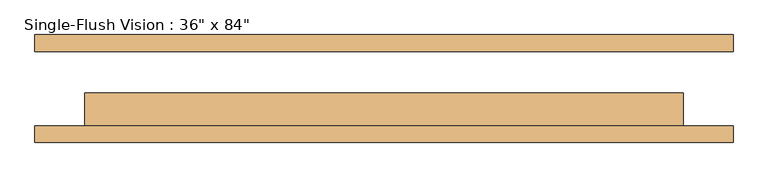
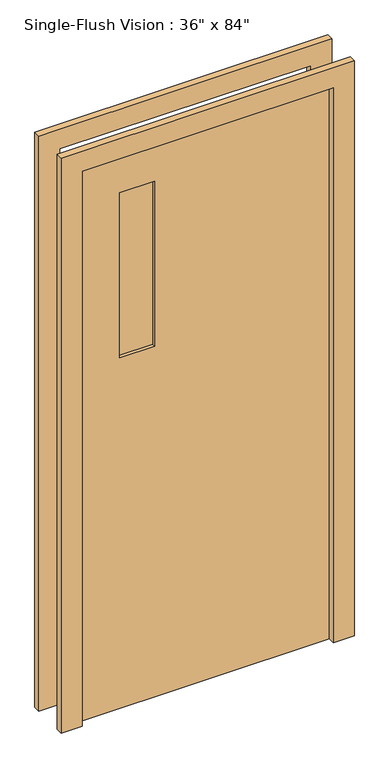
"""IFC4 building model written with IfcOpenShell, lengths in millimetres: door geometry."""

from ifc_helpers import new_model, si_unit, frame, origin, place, context, project, spatial, polyline, outline, extrude, source, transform, mapped, element, save


def door_2709d5e0(model_context):
    return source(origin(), model_context, "Body", "SweptSolid", [
        extrude(outline(polyline([(2209.8, -533.4), (0.0, -533.4), (0.0, -457.2), (2133.6, -457.2), (2133.6, 457.2), (0.0, 457.2), (0.0, 533.4), (2209.8, 533.4), (2209.8, -533.4)])), frame((0.0, -82.55, 0.0), z_axis=(0.0, 1.0, 0.0), x_axis=(0.0, 0.0, 1.0)), (0.0, 0.0, 1.0), 25.4),
        extrude(outline(polyline([(2133.6, 457.2), (0.0, 457.2), (0.0, 533.4), (2209.8, 533.4), (2209.8, -533.4), (0.0, -533.4), (0.0, -457.2), (2133.6, -457.2), (2133.6, 457.2)])), frame((0.0, 57.15, 0.0), z_axis=(0.0, 1.0, 0.0), x_axis=(0.0, 0.0, 1.0)), (0.0, 0.0, 1.0), 25.4),
        extrude(outline(polyline([(-177.8, -19.05), (-177.8, -25.4), (-304.8, -25.4), (-304.8, -19.05), (-177.8, -19.05)])), frame((0.0, 0.0, 1346.2), z_axis=(0.0, 0.0, 1.0), x_axis=(1.0, 0.0, 0.0)), (0.0, 0.0, 1.0), 635.0),
        extrude(outline(polyline([(-177.8, -38.1), (-177.8, -44.45), (-304.8, -44.45), (-304.8, -38.1), (-177.8, -38.1)])), frame((0.0, 0.0, 1346.2), z_axis=(0.0, 0.0, 1.0), x_axis=(1.0, 0.0, 0.0)), (0.0, 0.0, 1.0), 635.0),
        extrude(outline(polyline([(2133.6, -457.2), (0.0, -457.2), (0.0, 457.2), (2133.6, 457.2), (2133.6, -457.2)]), holes=[polyline([(1981.2, -304.8), (1981.2, -177.8), (1346.2, -177.8), (1346.2, -304.8), (1981.2, -304.8)])]), frame((0.0, -57.15, 0.0), z_axis=(0.0, 1.0, 0.0), x_axis=(0.0, 0.0, 1.0)), (0.0, 0.0, 1.0), 50.8),
    ])


if __name__ == "__main__":
    model = new_model("IFC4")
    model_context = context("Model", 3, world=origin())
    ifc_project = project(units=[si_unit("LENGTHUNIT", "METRE", prefix="MILLI")], contexts=[model_context])
    site = spatial("IfcSite", under=ifc_project)
    building = spatial("IfcBuilding", under=site)
    placement = place(None, origin())
    door_shape = door_2709d5e0(model_context)
    element("IfcDoor", 1, ObjectType="Single-Flush Vision : 36\" x 84\"", at=placement, inside=building, context=model_context, shape_type="MappedRepresentation", body=[
        mapped(door_shape, transform((0.0, 0.0, 0.0), x_axis=(1.0, 0.0, 0.0), y_axis=(0.0, 1.0, 0.0), z_axis=(0.0, 0.0, 1.0))),
    ])
    save(model, "model.ifc")

# Revit data of these elements
# Type "Single-Flush Vision : 36\" x 84\""
#   Type Mark = "21"
#   Assembly Code = "C1020"
#   Thickness = 0' - 2"
#   Height = 7' - 0"
#   Lite Height = 2' - 1"
#   Lite Width = 0' - 5"
#   Side Rail = 0' - 6"
#   Top Rail = 0' - 6"
#   Trim Projection = 0' - 1"
#   Trim Width Ext. = 0' - 3"
#   Trim Width Int. = 0' - 3"
#   Width = 3' - 0"
#   Function = 0
#   Door Material = Door - Panel
#   Frame Material = Door - Frame
#   Wall Closure = (empty or 0)
# Element 1 (IfcDoor, "Single-Flush Vision : 36\" x 84\"")
#   Materials on its faces: "Door - Frame", "Glass", "Door - Panel"
# Materials
#   "Door - Panel": class "Wood", colour RGB 230 193 158, transparency 0, Cost = 0
#   "Door - Frame": class "Paint", colour RGB 113 0 0, transparency 0, Cost = 0
#   "Glass": class "Glass", colour RGB 0 128 192, transparency 0.75, Cost = 0
